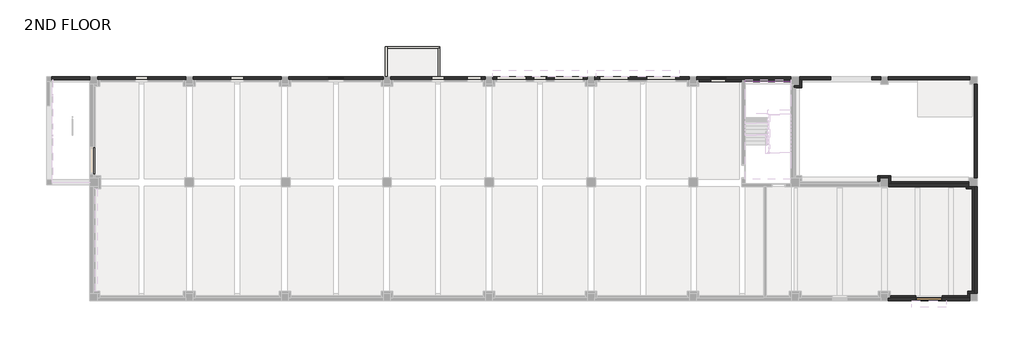
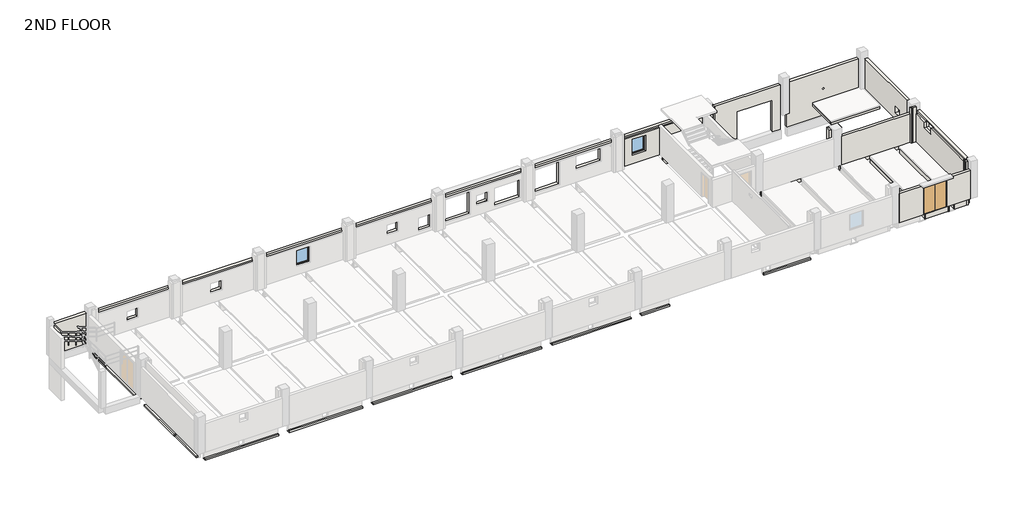
# One storey, part 3 of 7: 46 walls, 2 slabs, 2 windows, 1 door.
"""IFC4 building model written with IfcOpenShell, lengths in millimetres."""

import ifcopenshell
import ifcopenshell.guid

model = None  # the IFC model being written
_history = None  # IfcOwnerHistory: only IFC2X3 demands one
_inside = {}  # id of a spatial element -> (the spatial element, [elements in it])
_under = {}  # id of a project, library or spatial element -> (it, [spatial elements below it])
_declared = {}  # id of a project -> (the project, [libraries it declares])
_typed = {}  # id of a type object -> (the type object, [elements of that type])
_made_of = {}  # id of a material, layer set ... -> (it, [elements and type objects made of it])


def new_model(schema):
    """Start an empty IFC model of exactly this schema.

    Asked for "IFC4X3", IfcOpenShell would pick the latest addendum, in which some entities
    have other attributes; the version numbers below select the first issue.
    IFC2X3 requires an IfcOwnerHistory on every rooted entity: one is made here for all.
    """
    global model, _history
    if schema == "IFC4X3":
        model = ifcopenshell.file(schema_version=(4, 3, 0, 0))
    else:
        model = ifcopenshell.file(schema=schema)
    _inside.clear()
    _under.clear()
    _declared.clear()
    _typed.clear()
    _made_of.clear()
    _history = None
    if model.schema == "IFC2X3":
        org = make("IfcOrganization", Name="unknown")
        user = make(
            "IfcPersonAndOrganization",
            ThePerson=make("IfcPerson", FamilyName="unknown"),
            TheOrganization=org,
        )
        app = make(
            "IfcApplication",
            ApplicationDeveloper=org,
            Version="unknown",
            ApplicationFullName="unknown",
            ApplicationIdentifier="unknown",
        )
        _history = make(
            "IfcOwnerHistory",
            OwningUser=user,
            OwningApplication=app,
            ChangeAction="ADDED",
            CreationDate=0,
        )
    return model


def make(cls, **values):
    """One entity of the class cls with the attributes given. An attribute that is None is left unset."""
    return model.create_entity(
        cls, **{name: value for name, value in values.items() if value is not None}
    )


def rooted(cls, **values):
    """An entity with a GlobalId (a new one), such as an element, a storey or a relation."""
    return make(cls, GlobalId=ifcopenshell.guid.new(), OwnerHistory=_history, **values)


def si_unit(unit_type, name, prefix=None):
    """IfcSIUnit, for example si_unit("LENGTHUNIT", "METRE", prefix="MILLI")."""
    return make("IfcSIUnit", UnitType=unit_type, Prefix=prefix, Name=name)


def assignment(units):
    """IfcUnitAssignment: the units of a project."""
    return None if units is None else make("IfcUnitAssignment", Units=units)


def point(xyz):
    """IfcCartesianPoint."""
    return None if xyz is None else make("IfcCartesianPoint", Coordinates=xyz)


def direction(xyz):
    """IfcDirection."""
    return None if xyz is None else make("IfcDirection", DirectionRatios=xyz)


def frame(location, z_axis=None, x_axis=None):
    """IfcAxis2Placement3D, a coordinate frame: its origin and axes. An axis left out is left unset."""
    return make(
        "IfcAxis2Placement3D",
        Location=point(location),
        Axis=direction(z_axis),
        RefDirection=direction(x_axis),
    )


def frame_2d(location, x_axis=None):
    """IfcAxis2Placement2D, a coordinate frame in the plane: its origin and x axis."""
    return make(
        "IfcAxis2Placement2D", Location=point(location), RefDirection=direction(x_axis)
    )


def origin():
    """The frame at (0, 0, 0) with its axes left unset."""
    return frame((0.0, 0.0, 0.0))


def place(relative_to, where):
    """IfcLocalPlacement: puts the frame where relative to a parent placement (None: the world)."""
    return make(
        "IfcLocalPlacement", PlacementRelTo=relative_to, RelativePlacement=where
    )


def context(
    kind, dimensions, precision=None, world=None, true_north=None, identifier=None
):
    """IfcGeometricRepresentationContext, for example the 3D "Model" context."""
    return make(
        "IfcGeometricRepresentationContext",
        ContextIdentifier=identifier,
        ContextType=kind,
        CoordinateSpaceDimension=dimensions,
        Precision=precision,
        WorldCoordinateSystem=world,
        TrueNorth=true_north,
    )


def project(units=None, contexts=None):
    """IfcProject with its units and contexts."""
    return rooted(
        "IfcProject",
        Name="project",
        RepresentationContexts=contexts,
        UnitsInContext=assignment(units),
    )


def spatial(cls, under=None, at=None, **own):
    """A site, building, storey or space (cls), placed at a placement, below another one or the project."""
    s = rooted(cls, ObjectPlacement=at, **own)
    if under is not None:
        _under.setdefault(under.id(), (under, []))[1].append(s)
    return s


def polyline(points):
    """IfcPolyline through the points."""
    return make("IfcPolyline", Points=[point(p) for p in points])


def circle_curve(where, radius):
    """IfcCircle in the frame where."""
    return make("IfcCircle", Position=where, Radius=radius)


def trimmed(basis, trim1, trim2, sense, master):
    """IfcTrimmedCurve: the piece of a basis curve between two trims."""
    return make(
        "IfcTrimmedCurve",
        BasisCurve=basis,
        Trim1=trim1,
        Trim2=trim2,
        SenseAgreement=sense,
        MasterRepresentation=master,
    )


def segment(curve, same_sense, transition):
    """IfcCompositeCurveSegment."""
    return make(
        "IfcCompositeCurveSegment",
        Transition=transition,
        SameSense=same_sense,
        ParentCurve=curve,
    )


def composite_curve(segments, self_intersect=None):
    """IfcCompositeCurve: segments joined end to end."""
    return make("IfcCompositeCurve", Segments=segments, SelfIntersect=self_intersect)


def outline(outer, holes=None, kind="AREA"):
    """IfcArbitraryClosedProfileDef: a profile drawn as a closed curve; with holes, ...WithVoids."""
    if holes is None:
        return make("IfcArbitraryClosedProfileDef", ProfileType=kind, OuterCurve=outer)
    return make(
        "IfcArbitraryProfileDefWithVoids",
        ProfileType=kind,
        OuterCurve=outer,
        InnerCurves=holes,
    )


def extrude(swept, where, along, depth):
    """IfcExtrudedAreaSolid: the profile swept, set in the frame where, extruded along a direction by depth."""
    return make(
        "IfcExtrudedAreaSolid",
        SweptArea=swept,
        Position=where,
        ExtrudedDirection=direction(along),
        Depth=depth,
    )


def faces_of(points, faces, orient=None, outer=None):
    """IfcFace entities. A face is a list of loops; a loop is a list of indices into points, from 0.

    orient and outer hold one flag for each loop. By default every Orientation is true, the
    first loop of a face is its IfcFaceOuterBound and the others are IfcFaceBound.
    """
    made = []
    for i, loops in enumerate(faces):
        bounds = []
        for j, loop in enumerate(loops):
            is_outer = j == 0 if outer is None else outer[i][j]
            bounds.append(
                make(
                    "IfcFaceOuterBound" if is_outer else "IfcFaceBound",
                    Bound=make("IfcPolyLoop", Polygon=[points[k] for k in loop]),
                    Orientation=True if orient is None else orient[i][j],
                )
            )
        made.append(make("IfcFace", Bounds=bounds))
    return made


def faceted_brep(points, faces, orient=None, outer=None, voids=None):
    """IfcFacetedBrep: a solid bounded by flat faces; with voids (closed shells), ...WithVoids."""
    shared = [point(p) for p in points]
    hull = make("IfcClosedShell", CfsFaces=faces_of(shared, faces, orient, outer))
    if voids is None:
        return make("IfcFacetedBrep", Outer=hull)
    return make(
        "IfcFacetedBrepWithVoids",
        Outer=hull,
        Voids=[
            make(cls, CfsFaces=faces_of(shared, fs, o, b)) for cls, fs, o, b in voids
        ],
    )


def shape(context_of_items, identifier, shape_type, items):
    """IfcShapeRepresentation: the items that make up one representation, for example the "Body"."""
    return make(
        "IfcShapeRepresentation",
        ContextOfItems=context_of_items,
        RepresentationIdentifier=identifier,
        RepresentationType=shape_type,
        Items=items,
    )


def source(mapping_origin, context_of_items, identifier, shape_type, items):
    """IfcRepresentationMap: a shape defined once, which mapped items show again and again."""
    return make(
        "IfcRepresentationMap",
        MappingOrigin=mapping_origin,
        MappedRepresentation=shape(context_of_items, identifier, shape_type, items),
    )


def transform(
    local_origin,
    x_axis=None,
    y_axis=None,
    z_axis=None,
    scale=None,
    scale2=None,
    scale3=None,
    uniform=True,
):
    """IfcCartesianTransformationOperator3D, or its non-uniform kind. x_axis, y_axis, z_axis: its Axis1, 2, 3."""
    if uniform:
        return make(
            "IfcCartesianTransformationOperator3D",
            Axis1=direction(x_axis),
            Axis2=direction(y_axis),
            LocalOrigin=point(local_origin),
            Scale=scale,
            Axis3=direction(z_axis),
        )
    return make(
        "IfcCartesianTransformationOperator3DnonUniform",
        Axis1=direction(x_axis),
        Axis2=direction(y_axis),
        LocalOrigin=point(local_origin),
        Scale=scale,
        Axis3=direction(z_axis),
        Scale2=scale2,
        Scale3=scale3,
    )


def mapped(mapping_source, mapping_target):
    """IfcMappedItem: shows the shape of a source again, moved by a transform."""
    return make(
        "IfcMappedItem", MappingSource=mapping_source, MappingTarget=mapping_target
    )


def made_of(thing, what):
    """Note that an element or type object is made of a material, layer set ...; save() writes the relation."""
    if what is not None:
        _made_of.setdefault(what.id(), (what, []))[1].append(thing)
    return thing


def element(
    cls,
    number,
    at=None,
    inside=None,
    cuts=None,
    type_object=None,
    material=None,
    context=None,
    identifier="Body",
    shape_type=None,
    held_by="IfcProductDefinitionShape",
    body=None,
    shapes=None,
    **own,
):
    """One element of the class cls, such as IfcWall. Its Tag is "e" and its number.

    at: its placement. inside: the storey or other place that contains it. cuts: it is an
    opening in that element (IfcRelVoidsElement). A single representation is given by context,
    identifier, shape_type and body (its items); several are given by shapes. held_by: the class
    of the entity that holds the representations. save() writes the other relations.
    """
    e = rooted(cls, Tag="e%d" % number, ObjectPlacement=at, **own)
    if body is not None:
        shapes = [shape(context, identifier, shape_type, body)]
    if shapes is not None:
        e.Representation = make(held_by, Representations=shapes)
    if inside is not None:
        _inside.setdefault(inside.id(), (inside, []))[1].append(e)
    if cuts is not None:
        rooted(
            "IfcRelVoidsElement", RelatingBuildingElement=cuts, RelatedOpeningElement=e
        )
    if type_object is not None:
        _typed.setdefault(type_object.id(), (type_object, []))[1].append(e)
    return made_of(e, material)


def aggregate(whole, parts):
    """IfcRelAggregates: a whole, such as a stair, and the parts it consists of."""
    return rooted("IfcRelAggregates", RelatingObject=whole, RelatedObjects=parts)


def save(model, path):
    """Write the relations noted so far, then the file.

    IfcRelAggregates (storeys below a building ...), IfcRelContainedInSpatialStructure (elements
    in a storey), IfcRelDefinesByType, IfcRelAssociatesMaterial and IfcRelDeclares: one each for
    every whole, place, type object, material and project.
    """
    for whole, parts in _under.values():
        aggregate(whole, parts)
    for where, things in _inside.values():
        rooted(
            "IfcRelContainedInSpatialStructure",
            RelatedElements=things,
            RelatingStructure=where,
        )
    for kind, things in _typed.values():
        rooted("IfcRelDefinesByType", RelatedObjects=things, RelatingType=kind)
    for what, things in _made_of.values():
        rooted("IfcRelAssociatesMaterial", RelatedObjects=things, RelatingMaterial=what)
    for by, libraries in _declared.values():
        rooted("IfcRelDeclares", RelatingContext=by, RelatedDefinitions=libraries)
    model.write(path)


def plane_surface(at):
    """IfcPlane: the flat surface through the origin of the frame at, square to its z axis."""
    return make("IfcPlane", Position=at)


def revolved_surface(curve, axis_point, axis_direction):
    """IfcSurfaceOfRevolution: the curve turned about the line through axis_point along axis_direction."""
    return make(
        "IfcSurfaceOfRevolution",
        SweptCurve=make("IfcArbitraryOpenProfileDef", ProfileType="CURVE", Curve=curve),
        AxisPosition=make("IfcAxis1Placement", Location=point(axis_point), Axis=direction(axis_direction)),
    )


def advanced_brep(points, edges, surfaces, faces):
    """IfcAdvancedBrep: a solid bounded by faces that lie on surfaces and meet in shared edges.

    An edge is (start, end): straight between two places in points (the first is 0);
    or (start, end, curve); or (start, end, curve, False) where it runs against its curve.
    A face is (place in surfaces, loops), or (place, loops, False) where it looks against
    its surface's normal. A loop lists edges by number (the first is 1), with a minus sign
    where the edge is run from its end to its start. The first loop is the outer one.
    """
    corners = [point(p) for p in points]
    vertices = [make("IfcVertexPoint", VertexGeometry=c) for c in corners]
    made = []
    for start, end, *more in edges:
        made.append(
            make(
                "IfcEdgeCurve",
                EdgeStart=vertices[start],
                EdgeEnd=vertices[end],
                EdgeGeometry=more[0] if more else make("IfcPolyline", Points=[corners[start], corners[end]]),
                SameSense=more[1] if len(more) > 1 else True,
            )
        )
    hull = []
    for where, loops, *sense in faces:
        bounds = []
        for j, loop in enumerate(loops):
            ring = [make("IfcOrientedEdge", EdgeElement=made[abs(k) - 1], Orientation=k > 0) for k in loop]
            bounds.append(
                make(
                    "IfcFaceOuterBound" if j == 0 else "IfcFaceBound",
                    Bound=make("IfcEdgeLoop", EdgeList=ring),
                    Orientation=True,
                )
            )
        hull.append(make("IfcAdvancedFace", Bounds=bounds, FaceSurface=surfaces[where], SameSense=sense[0] if sense else True))
    return make("IfcAdvancedBrep", Outer=make("IfcClosedShell", CfsFaces=hull))


def double_door_steel_c24d22a6(model_context):
    return source(origin(), model_context, "Body", "SolidModel", [
        faceted_brep([(-1035.0, -125.0, 2565.0), (-1035.0, 125.0, 2565.0), (-1035.0, 125.0, 0.0), (-1035.0, -125.0, 0.0), (1035.0, 125.0, 0.0), (1035.0, 125.0, 2565.0), (1005.0, 125.0, 2535.0), (-1005.0, 125.0, 2535.0), (-1005.0, 125.0, 30.0), (1005.0, 125.0, 30.0), (1035.0, -125.0, 0.0), (1035.0, -125.0, 2565.0), (1005.0, -125.0, 30.0), (-1005.0, -125.0, 30.0), (-1005.0, -125.0, 2535.0), (1005.0, -125.0, 2535.0), (-1005.0, -85.0, 2535.0), (-1005.0, -85.0, 30.0), (1005.0, -85.0, 30.0), (1005.0, -85.0, 2535.0), (985.0, -85.0, 2515.0), (985.0, -85.0, 50.0), (-985.0, -85.0, 50.0), (-985.0, -85.0, 2515.0), (-985.0, 85.0, 2515.0), (-985.0, 85.0, 50.0), (985.0, 85.0, 50.0), (1005.0, 85.0, 30.0), (-1005.0, 85.0, 30.0), (-1005.0, 85.0, 2535.0), (1005.0, 85.0, 2535.0), (985.0, 85.0, 2515.0)], [[[0, 1, 2, 3]], [[4, 2, 1, 5], [6, 7, 8, 9]], [[3, 2, 4, 10]], [[11, 0, 3, 10], [12, 13, 14, 15]], [[16, 14, 13, 17]], [[17, 13, 12, 18]], [[16, 17, 18, 19], [20, 21, 22, 23]], [[24, 23, 22, 25]], [[25, 22, 21, 26]], [[27, 28, 29, 30], [31, 24, 25, 26]], [[7, 29, 28, 8]], [[8, 28, 27, 9]], [[10, 4, 5, 11]], [[9, 27, 30, 6]], [[18, 12, 15, 19]], [[26, 21, 20, 31]], [[11, 5, 1, 0]], [[19, 15, 14, 16]], [[31, 20, 23, 24]], [[6, 30, 29, 7]]]),
        extrude(outline(polyline([(1005.0, 85.0), (0.0, 85.0), (0.0, 125.0), (1005.0, 125.0), (1005.0, 85.0)])), frame((0.0, 0.0, 30.0), z_axis=(0.0, 0.0, 1.0), x_axis=(1.0, 0.0, 0.0)), (0.0, 0.0, 1.0), 2505.0),
        extrude(outline(polyline([(0.0, 85.0), (-1005.0, 85.0), (-1005.0, 125.0), (0.0, 125.0), (0.0, 85.0)])), frame((0.0, 0.0, 30.0), z_axis=(0.0, 0.0, 1.0), x_axis=(1.0, 0.0, 0.0)), (0.0, 0.0, 1.0), 2505.0),
    ])


def fixed_window_c6e05aa5(model_context):
    return source(origin(), model_context, "Body", "SweptSolid", [
        extrude(outline(polyline([(-550.0, 3.0), (550.0, 3.0), (550.0, -3.0), (-550.0, -3.0), (-550.0, 3.0)])), frame((0.0, 0.0, 850.0), z_axis=(0.0, 0.0, 1.0), x_axis=(1.0, 0.0, 0.0)), (0.0, 0.0, 1.0), 1400.0),
        extrude(outline(polyline([(2300.0, -600.0), (800.0, -600.0), (800.0, 600.0), (2300.0, 600.0), (2300.0, -600.0)]), holes=[polyline([(2250.0, -550.0), (2250.0, 550.0), (850.0, 550.0), (850.0, -550.0), (2250.0, -550.0)])]), frame((0.0, -75.0, 0.0), z_axis=(0.0, 1.0, 0.0), x_axis=(0.0, 0.0, 1.0)), (0.0, 0.0, 1.0), 150.0),
    ])


model = new_model("IFC4")

# Units and contexts
model_context = context("Model", 3, world=origin())
ifc_project = project(units=[si_unit("LENGTHUNIT", "METRE", prefix="MILLI")], contexts=[model_context])

# Site, building, storey
site = spatial("IfcSite", under=ifc_project)
building = spatial("IfcBuilding", under=site)
storey = spatial("IfcBuildingStorey", under=building, Name="2ND FLOOR", Elevation=10600.0)

# Door
placement = place(None, origin())
double_door_steel_shape = double_door_steel_c24d22a6(model_context)
element("IfcDoor", 1, ObjectType="Double Door_Steel : H_DR_AR B12_Door_Double_W2100xH2580_No FR_SD-5", at=placement, inside=storey, context=model_context, shape_type="MappedRepresentation", body=[
    mapped(double_door_steel_shape, transform((65500.0, -17175.0, 10600.0), x_axis=(-1.0, 0.0, 0.0), y_axis=(0.0, -1.0, 0.0), z_axis=(0.0, 0.0, 1.0))),
])

# Slabs
element("IfcSlab", 2, ObjectType="H_WA_AR_B02_Int Wall_2L Gypsum_Insulationl_T154(Mirror)", at=placement, inside=storey, context=model_context, shape_type="Brep", body=[
    faceted_brep([(264.0, -8514.0, 9736.0), (264.0, -13136.0, 9736.0), (114.0, -13136.0, 9736.0), (-40.0, -13136.0, 9736.0), (-40.0, -8514.0, 9736.0), (114.0, -8514.0, 9736.0), (110.0, -8514.0, 9890.0), (-40.0, -8514.0, 9890.0), (-40.0, -13136.0, 9890.0), (110.0, -13136.0, 9890.0), (264.0, -8514.0, 9755.0), (264.0, -13136.0, 9755.0), (110.0, -8514.0, 9755.0), (110.0, -13136.0, 9755.0), (114.0, -13136.0, 9755.0), (-40.0, -13136.0, 9755.0)], [[[0, 1, 2, 3, 4, 5]], [[6, 7, 8, 9]], [[1, 0, 10, 11]], [[0, 5, 4, 7, 6, 12, 10]], [[13, 12, 6, 9]], [[12, 13, 14, 11, 10]], [[3, 2, 1, 11, 14, 13, 9, 8, 15]], [[4, 3, 15, 8, 7]]]),
    faceted_brep([(264.0, -16536.0, 9736.0), (114.0, -16536.0, 9736.0), (-40.0, -16536.0, 9736.0), (-40.0, -13264.0, 9736.0), (114.0, -13264.0, 9736.0), (264.0, -13264.0, 9736.0), (-40.0, -13264.0, 9890.0), (-40.0, -16536.0, 9890.0), (110.0, -16536.0, 9890.0), (110.0, -13264.0, 9890.0), (264.0, -16536.0, 9755.0), (110.0, -16536.0, 9755.0), (-40.0, -13264.0, 9755.0), (110.0, -13264.0, 9755.0), (264.0, -13264.0, 9755.0), (114.0, -13264.0, 9755.0)], [[[0, 1, 2, 3, 4, 5]], [[6, 7, 8, 9]], [[2, 1, 0, 10, 11, 8, 7]], [[3, 2, 7, 6, 12]], [[9, 8, 11, 13]], [[14, 15, 13, 11, 10]], [[5, 4, 3, 12, 6, 9, 13, 15, 14]], [[0, 5, 14, 10]]]),
    faceted_brep([(264.0, -7486.0, 9736.0), (114.0, -7486.0, 9736.0), (-40.0, -7486.0, 9736.0), (-40.0, -464.0, 9736.0), (114.0, -464.0, 9736.0), (264.0, -464.0, 9736.0), (-40.0, -464.0, 9890.0), (-40.0, -7486.0, 9890.0), (110.0, -7486.0, 9890.0), (110.0, -464.0, 9890.0), (264.0, -7486.0, 9755.0), (110.0, -7486.0, 9755.0), (110.0, -464.0, 9755.0), (264.0, -464.0, 9755.0)], [[[0, 1, 2, 3, 4, 5]], [[6, 7, 8, 9]], [[2, 1, 0, 10, 11, 8, 7]], [[3, 2, 7, 6]], [[5, 4, 3, 6, 9, 12, 13]], [[0, 5, 13, 10]], [[11, 12, 9, 8]], [[12, 11, 10, 13]]]),
])
element("IfcSlab", 3, ObjectType="H_WA_AR_B02_Int Wall_2L Gypsum_Insulationl_T154(Mirror)", at=placement, inside=storey, context=model_context, shape_type="Brep", body=[
    faceted_brep([(464.0, -17040.0, 9636.0), (464.0, -16886.0, 9636.0), (464.0, -16736.0, 9636.0), (7036.0, -16736.0, 9636.0), (7036.0, -16886.0, 9636.0), (7036.0, -17040.0, 9636.0), (464.0, -17040.0, 9790.0), (7036.0, -17040.0, 9790.0), (7036.0, -16890.0, 9790.0), (464.0, -16890.0, 9790.0), (464.0, -16890.0, 9655.0), (464.0, -16736.0, 9655.0), (7036.0, -16736.0, 9655.0), (7036.0, -16890.0, 9655.0)], [[[0, 1, 2, 3, 4, 5]], [[6, 7, 8, 9]], [[2, 1, 0, 6, 9, 10, 11]], [[3, 2, 11, 12]], [[5, 4, 3, 12, 13, 8, 7]], [[0, 5, 7, 6]], [[13, 10, 9, 8]], [[10, 13, 12, 11]]]),
    faceted_brep([(14536.0, -16736.0, 9636.0), (14536.0, -16886.0, 9636.0), (14536.0, -17040.0, 9636.0), (7964.0, -17040.0, 9636.0), (7964.0, -16886.0, 9636.0), (7964.0, -16736.0, 9636.0), (7964.0, -17040.0, 9790.0), (14536.0, -17040.0, 9790.0), (14536.0, -16890.0, 9790.0), (7964.0, -16890.0, 9790.0), (14536.0, -16736.0, 9655.0), (14536.0, -16890.0, 9655.0), (7964.0, -16890.0, 9655.0), (7964.0, -16736.0, 9655.0)], [[[0, 1, 2, 3, 4, 5]], [[6, 7, 8, 9]], [[2, 1, 0, 10, 11, 8, 7]], [[3, 2, 7, 6]], [[5, 4, 3, 6, 9, 12, 13]], [[0, 5, 13, 10]], [[11, 12, 9, 8]], [[12, 11, 10, 13]]]),
    faceted_brep([(23464.0, -16736.0, 9636.0), (30536.0, -16736.0, 9636.0), (30536.0, -16886.0, 9636.0), (23464.0, -16886.0, 9636.0), (23464.0, -16736.0, 9655.0), (23464.0, -16886.0, 9655.0), (30536.0, -16736.0, 9655.0), (30536.0, -16886.0, 9655.0)], [[[0, 1, 2, 3]], [[4, 0, 3, 5]], [[1, 0, 4, 6]], [[2, 1, 6, 7]], [[6, 4, 5, 7]], [[3, 2, 7, 5]]]),
    faceted_brep([(31464.0, -16736.0, 9636.0), (38536.0, -16736.0, 9636.0), (38536.0, -16886.0, 9636.0), (31464.0, -16886.0, 9636.0), (31464.0, -16736.0, 9655.0), (31464.0, -16886.0, 9655.0), (38536.0, -16736.0, 9655.0), (38536.0, -16886.0, 9655.0)], [[[0, 1, 2, 3]], [[4, 0, 3, 5]], [[1, 0, 4, 6]], [[1, 6, 7, 2]], [[6, 4, 5, 7]], [[3, 2, 7, 5]]]),
    faceted_brep([(22536.0, -17040.0, 9636.0), (15464.0, -17040.0, 9636.0), (15464.0, -16886.0, 9636.0), (15464.0, -16736.0, 9636.0), (22536.0, -16736.0, 9636.0), (22536.0, -16886.0, 9636.0), (15464.0, -17040.0, 9790.0), (22536.0, -17040.0, 9790.0), (22536.0, -16890.0, 9790.0), (15464.0, -16890.0, 9790.0), (15464.0, -16890.0, 9655.0), (15464.0, -16736.0, 9655.0), (22536.0, -16736.0, 9655.0), (22536.0, -16890.0, 9655.0)], [[[0, 1, 2, 3, 4, 5]], [[6, 7, 8, 9]], [[1, 0, 7, 6]], [[3, 2, 1, 6, 9, 10, 11]], [[4, 3, 11, 12]], [[0, 5, 4, 12, 13, 8, 7]], [[13, 10, 9, 8]], [[10, 13, 12, 11]]]),
    faceted_brep([(41975.0, -16736.0, 9636.0), (41975.0, -16886.0, 9636.0), (41975.0, -17040.0, 9636.0), (39464.0, -17040.0, 9636.0), (39464.0, -16886.0, 9636.0), (39464.0, -16736.0, 9636.0), (39464.0, -17040.0, 9790.0), (41975.0, -17040.0, 9790.0), (41975.0, -16890.0, 9790.0), (39464.0, -16890.0, 9790.0), (41975.0, -16736.0, 9655.0), (41975.0, -16890.0, 9655.0), (39464.0, -16890.0, 9655.0), (39464.0, -16736.0, 9655.0)], [[[0, 1, 2, 3, 4, 5]], [[6, 7, 8, 9]], [[2, 1, 0, 10, 11, 8, 7]], [[3, 2, 7, 6]], [[5, 4, 3, 6, 9, 12, 13]], [[0, 5, 13, 10]], [[11, 12, 9, 8]], [[12, 11, 10, 13]]]),
    faceted_brep([(50343.0, -16736.0, 9636.0), (54536.0, -16736.0, 9636.0), (54536.0, -16886.0, 9636.0), (54536.0, -17040.0, 9636.0), (50343.0, -17040.0, 9636.0), (50343.0, -16886.0, 9636.0), (50343.0, -17040.0, 9790.0), (54536.0, -17040.0, 9790.0), (54536.0, -16890.0, 9790.0), (50343.0, -16890.0, 9790.0), (50343.0, -16736.0, 9655.0), (54536.0, -16736.0, 9655.0), (54536.0, -16890.0, 9655.0), (50343.0, -16890.0, 9655.0)], [[[0, 1, 2, 3, 4, 5]], [[6, 7, 8, 9]], [[1, 0, 10, 11]], [[3, 2, 1, 11, 12, 8, 7]], [[4, 3, 7, 6]], [[0, 5, 4, 6, 9, 13, 10]], [[12, 13, 9, 8]], [[13, 12, 11, 10]]]),
    faceted_brep([(23464.0, -17040.0, 9790.0), (30536.0, -17040.0, 9790.0), (30536.0, -16890.0, 9790.0), (23464.0, -16890.0, 9790.0), (23464.0, -16890.0, 9655.0), (23464.0, -17040.0, 9655.0), (30536.0, -17040.0, 9655.0), (30536.0, -16890.0, 9655.0)], [[[0, 1, 2, 3]], [[0, 3, 4, 5]], [[1, 6, 7, 2]], [[1, 0, 5, 6]], [[3, 2, 7, 4]], [[5, 4, 7, 6]]]),
    faceted_brep([(31464.0, -17040.0, 9790.0), (38536.0, -17040.0, 9790.0), (38536.0, -16890.0, 9790.0), (31464.0, -16890.0, 9790.0), (31464.0, -17040.0, 9655.0), (38536.0, -17040.0, 9655.0), (31464.0, -16890.0, 9655.0), (38536.0, -16890.0, 9655.0)], [[[0, 1, 2, 3]], [[1, 0, 4, 5]], [[0, 3, 6, 4]], [[2, 1, 5, 7]], [[3, 2, 7, 6]], [[5, 4, 6, 7]]]),
])

# Walls
element("IfcWall", 4, ObjectType="H_WA_AR B02_Ext Wall RC-AG_T250_W1", at=placement, inside=storey, context=model_context, shape_type="SweptSolid", body=[
    extrude(outline(polyline([(10600.0, 300.0), (10600.0, 7200.0), (13300.0, 7200.0), (13300.0, 300.0), (10600.0, 300.0)]), holes=[polyline([(12450.0, 3250.0), (12450.0, 4250.0), (11550.0, 4250.0), (11550.0, 3250.0), (12450.0, 3250.0)])]), frame((0.0, 50.0, 0.0), z_axis=(0.0, 1.0, 0.0), x_axis=(0.0, 0.0, 1.0)), (0.0, 0.0, 1.0), 250.0),
])
element("IfcWall", 5, ObjectType="H_WA_AR B02_Ext Wall RC-AG_T250_W1", at=placement, inside=storey, context=model_context, shape_type="SweptSolid", body=[
    extrude(outline(polyline([(10600.0, 7800.0), (10600.0, 14700.0), (13300.0, 14700.0), (13300.0, 7800.0), (10600.0, 7800.0)]), holes=[polyline([(12450.0, 10750.0), (12450.0, 11750.0), (11550.0, 11750.0), (11550.0, 10750.0), (12450.0, 10750.0)])]), frame((0.0, 50.0, 0.0), z_axis=(0.0, 1.0, 0.0), x_axis=(0.0, 0.0, 1.0)), (0.0, 0.0, 1.0), 250.0),
])
element("IfcWall", 6, ObjectType="H_WA_AR B02_Ext Wall RC-AG_T250_W1", at=placement, inside=storey, context=model_context, shape_type="SweptSolid", body=[
    extrude(outline(polyline([(10600.0, 15299.9999999), (10600.0, 22700.0), (13300.0, 22700.0), (13300.0, 15299.9999999), (10600.0, 15299.9999999)]), holes=[polyline([(11400.0, 19599.9999999), (11400.0, 18399.9999999), (12900.0, 18399.9999999), (12900.0, 19599.9999999), (11400.0, 19599.9999999)])]), frame((0.0, 50.0, 0.0), z_axis=(0.0, 1.0, 0.0), x_axis=(0.0, 0.0, 1.0)), (0.0, 0.0, 1.0), 250.0),
])
element("IfcWall", 7, ObjectType="H_WA_AR B02_Ext Wall RC-AG_T250_W1", at=placement, inside=storey, context=model_context, shape_type="SweptSolid", body=[
    extrude(outline(polyline([(10600.0, 23300.0), (10600.0, 30700.0), (13300.0, 30700.0), (13300.0, 23300.0), (10600.0, 23300.0)]), holes=[polyline([(12150.0, 29300.0), (12150.0, 30400.0), (10900.0, 30400.0), (10900.0, 29300.0), (12150.0, 29300.0)]), polyline([(12450.0, 26500.0), (12450.0, 27500.0), (11550.0, 27500.0), (11550.0, 26500.0), (12450.0, 26500.0)])]), frame((0.0, 50.0, 0.0), z_axis=(0.0, 1.0, 0.0), x_axis=(0.0, 0.0, 1.0)), (0.0, 0.0, 1.0), 250.0),
])
element("IfcWall", 8, ObjectType="H_WA_AR B02_Ext Wall RC-AG_T250_W1", at=placement, inside=storey, context=model_context, shape_type="SweptSolid", body=[
    extrude(outline(polyline([(10600.0, 31300.0), (10600.0, 38700.0), (13300.0, 38700.0), (13300.0, 31300.0), (10600.0, 31300.0)]), holes=[polyline([(12600.0, 36100.0), (12600.0, 38400.0), (10900.0, 38400.0), (10900.0, 36100.0), (12600.0, 36100.0)]), polyline([(13050.0, 31600.0), (13050.0, 33900.0), (10900.0, 33900.0), (10900.0, 31600.0), (13050.0, 31600.0)]), polyline([(12450.0, 34500.0), (12450.0, 35500.0), (11550.0, 35500.0), (11550.0, 34500.0), (12450.0, 34500.0)])]), frame((0.0, 50.0, 0.0), z_axis=(0.0, 1.0, 0.0), x_axis=(0.0, 0.0, 1.0)), (0.0, 0.0, 1.0), 250.0),
])
element("IfcWall", 9, ObjectType="H_WA_AR B02_Ext Wall RC-AG_T250_W1", at=placement, inside=storey, context=model_context, shape_type="SweptSolid", body=[
    extrude(outline(polyline([(10600.0, 39300.0), (10600.0, 46700.0), (13300.0, 46700.0), (13300.0, 39300.0), (10600.0, 39300.0)]), holes=[composite_curve([segment(trimmed(circle_curve(frame_2d((12955.0, 46436.0)), 25.0), [point((12955.0, 46411.0))], [point((12955.0, 46461.0))], True, "CARTESIAN"), True, "CONTINUOUS"), segment(trimmed(circle_curve(frame_2d((12955.0, 46436.0)), 25.0), [point((12955.0, 46461.0))], [point((12955.0, 46411.0))], True, "CARTESIAN"), True, "CONTINUOUS")], self_intersect=False), polyline([(13050.0, 43400.0), (13050.0, 45600.0), (11800.0, 45600.0), (11800.0, 43400.0), (13050.0, 43400.0)]), polyline([(10900.0, 39700.0195059), (13050.0, 39700.0195059), (13050.0, 41900.0195059), (10900.0, 41900.0195059), (10900.0, 39700.0195059)])]), frame((0.0, 50.0, 0.0), z_axis=(0.0, 1.0, 0.0), x_axis=(0.0, 0.0, 1.0)), (0.0, 0.0, 1.0), 250.0),
])
element("IfcWall", 10, ObjectType="H_WA_AR B02_Ext Wall RC-AG_T250_W1", at=placement, inside=storey, context=model_context, shape_type="Brep", body=[
    faceted_brep([(47300.0, 50.0, 10600.0), (50825.0, 50.0, 10600.0), (51075.0, 50.0, 10600.0), (54650.0, 50.0, 10600.0), (54650.0, 50.0, 13300.0), (51075.0, 50.0, 13300.0), (50825.0, 50.0, 13300.0), (47300.0, 50.0, 13300.0), (49575.0, 50.0, 11400.0), (48375.0, 50.0, 11400.0), (48375.0, 50.0, 12900.0), (49575.0, 50.0, 12900.0), (47300.0, 300.0, 10600.0), (47300.0, 300.0, 13300.0), (54650.0, 300.0, 13300.0), (54650.0, 300.0, 10600.0), (49575.0, 300.0, 11400.0), (49575.0, 300.0, 12900.0), (48375.0, 300.0, 12900.0), (48375.0, 300.0, 11400.0)], [[[0, 1, 2, 3, 4, 5, 6, 7], [8, 9, 10, 11]], [[12, 13, 14, 15], [16, 17, 18, 19]], [[3, 2, 1, 0, 12, 15]], [[4, 3, 15, 14]], [[7, 6, 5, 4, 14, 13]], [[0, 7, 13, 12]], [[17, 16, 8, 11]], [[18, 17, 11, 10]], [[19, 18, 10, 9]], [[16, 19, 9, 8]]]),
])
element("IfcWall", 11, ObjectType="H_WA_AR B02_Ext Wall RC-AG_T250_W1", at=placement, inside=storey, context=model_context, shape_type="Brep", body=[
    faceted_brep([(61000.0, 50.0, 12100.0), (61000.0, 50.0, 9100.0), (61700.0, 50.0, 9100.0), (61700.0, 50.0, 13300.0), (55350.0, 50.0, 13300.0), (55350.0, 50.0, 9100.0), (57800.0, 50.0, 9100.0), (57800.0, 50.0, 12100.0), (61700.0, 300.0, 9100.0), (61000.0, 300.0, 9100.0), (61000.0, 300.0, 12100.0), (57800.0, 300.0, 12100.0), (57800.0, 300.0, 9100.0), (55350.0, 300.0, 9100.0), (55350.0, 300.0, 10600.0), (55350.0, 300.0, 13300.0), (61700.0, 300.0, 13300.0), (61700.0, 300.0, 10600.0)], [[[0, 1, 2, 3, 4, 5, 6, 7]], [[8, 9, 10, 11, 12, 13, 14, 15, 16, 17]], [[6, 5, 13, 12]], [[2, 1, 9, 8]], [[3, 2, 8, 17, 16]], [[4, 3, 16, 15]], [[5, 4, 15, 14, 13]], [[12, 11, 7, 6]], [[10, 9, 1, 0]], [[11, 10, 0, 7]]]),
])
element("IfcWall", 12, ObjectType="H_WA_AR B02_Ext Wall RC-AG_T250_W1", at=placement, inside=storey, context=model_context, shape_type="AdvancedBrep", body=[
    advanced_brep(
    [(62300.0, 50.0, 9100.0), (68700.0, 50.0, 9100.0), (68700.0, 50.0, 13300.0), (62300.0, 50.0, 13300.0), (65618.0, 50.0, 11600.0), (65468.0, 50.0, 11600.0), (68700.0, 300.0, 9100.0), (62300.0, 300.0, 9100.0), (62300.0, 300.0, 10600.0), (62300.0, 300.0, 13300.0), (68700.0, 300.0, 13300.0), (68700.0, 300.0, 10600.0), (65468.0, 300.0, 11600.0), (65618.0, 300.0, 11600.0)],
    [
        (0, 1),
        (1, 2),
        (2, 3),
        (3, 0),
        (4, 5, circle_curve(frame((65543.0, 50.0, 11600.0), z_axis=(0.0, 1.0, 0.0), x_axis=(1.0, 0.0, 0.0)), 75.0)),
        (5, 4, circle_curve(frame((65543.0, 50.0, 11600.0), z_axis=(0.0, 1.0, 0.0), x_axis=(1.0, 0.0, 0.0)), 75.0)),
        (6, 7),
        (7, 8),
        (8, 9),
        (9, 10),
        (10, 11),
        (11, 6),
        (12, 13, circle_curve(frame((65543.0, 300.0, 11600.0), z_axis=(0.0, -1.0, 0.0), x_axis=(1.0, 0.0, 0.0)), 75.0)),
        (13, 12, circle_curve(frame((65543.0, 300.0, 11600.0), z_axis=(0.0, -1.0, 0.0), x_axis=(1.0, 0.0, 0.0)), 75.0)),
        (0, 7),
        (6, 1),
        (10, 2),
        (9, 3),
        (12, 5),
        (4, 13),
    ],
    [
        plane_surface(frame((62300.0, 50.0, 9100.0), z_axis=(0.0, -1.0, 0.0), x_axis=(1.0, 0.0, 0.0))),
        plane_surface(frame((62300.0, 300.0, 9100.0), z_axis=(0.0, 1.0, 0.0), x_axis=(-1.0, 0.0, 0.0))),
        plane_surface(frame((62300.0, 50.0, 9100.0), z_axis=(0.0, 0.0, -1.0), x_axis=(0.0, 1.0, 0.0))),
        plane_surface(frame((68700.0, 50.0, 9100.0), z_axis=(1.0, 0.0, 0.0), x_axis=(0.0, 1.0, 0.0))),
        plane_surface(frame((68700.0, 50.0, 13300.0), z_axis=(0.0, 0.0, 1.0), x_axis=(0.0, 1.0, 0.0))),
        plane_surface(frame((62300.0, 50.0, 13300.0), z_axis=(-1.0, 0.0, 0.0), x_axis=(0.0, 1.0, 0.0))),
        revolved_surface(polyline([(65618.0, 50.0, 11600.0), (65618.0, 300.0, 11600.0)]), (65543.0, 50.0, 11600.0), (0.0, -1.0, 0.0)),
    ],
    [
        (0, [[1, 2, 3, 4], [5, 6]]),
        (1, [[7, 8, 9, 10, 11, 12], [13, 14]]),
        (2, [[-1, 15, -7, 16]]),
        (3, [[-2, -16, -12, -11, 17]]),
        (4, [[-3, -17, -10, 18]]),
        (5, [[-4, -18, -9, -8, -15]]),
        (6, [[-13, 19, -5, 20]]),
        (6, [[-14, -20, -6, -19]]),
    ],
),
])
element("IfcWall", 13, ObjectType="H_WA_AR B02_Ext Wall RC-AG_T250_W1", at=placement, inside=storey, context=model_context, shape_type="SweptSolid", body=[
    extrude(outline(polyline([(-300.0, 10600.0), (-7650.0, 10600.0), (-7650.0, 13400.0), (-300.0, 13400.0), (-300.0, 10600.0)]), holes=[polyline([(-5050.0, 11800.0), (-5650.0, 11800.0), (-5650.0, 11200.0), (-5050.0, 11200.0), (-5050.0, 11800.0)])]), frame((69050.0, 0.0, 0.0), z_axis=(1.0, 0.0, 0.0), x_axis=(0.0, 1.0, 0.0)), (0.0, 0.0, 1.0), 250.0),
])
element("IfcWall", 14, ObjectType="H_WA_AR B02_Ext Wall RC-AG_T250_W1", at=placement, inside=storey, context=model_context, shape_type="SweptSolid", body=[
    extrude(outline(polyline([(-8350.0, 10600.0), (-16700.0, 10600.0), (-16700.0, 13400.0), (-8350.0, 13400.0), (-8350.0, 10600.0)]), holes=[polyline([(-9800.0, 13300.0), (-10800.0, 13300.0), (-10800.0, 12700.0), (-9800.0, 12700.0), (-9800.0, 13300.0)])]), frame((69050.0, 0.0, 0.0), z_axis=(1.0, 0.0, 0.0), x_axis=(0.0, 1.0, 0.0)), (0.0, 0.0, 1.0), 250.0),
])
element("IfcWall", 15, ObjectType="H_WA_AR B02_Ext Wall RC-AG_T250_W1", at=placement, inside=storey, context=model_context, shape_type="SweptSolid", body=[
    extrude(outline(polyline([(13300.0, 62300.0), (10600.0, 62300.0), (10600.0, 64450.0), (13180.0, 64450.0), (13180.0, 66550.0), (10600.0, 66550.0), (10600.0, 68700.0), (13300.0, 68700.0), (13300.0, 62300.0)])), frame((0.0, -17300.0, 0.0), z_axis=(0.0, 1.0, 0.0), x_axis=(0.0, 0.0, 1.0)), (0.0, 0.0, 1.0), 250.0),
])
element("IfcWall", 16, ObjectType="H_WA_AR B02_Ext Wall RC-AG_T250_W1", at=placement, inside=storey, context=model_context, shape_type="Brep", body=[
    faceted_brep([(-300.0, 300.0, 10550.0), (-3300.0, 300.0, 10550.0), (-3300.0, 300.0, 10600.0), (-3300.0, 300.0, 13450.0), (-300.0, 300.0, 13450.0), (-300.0, 300.0, 10600.0), (-300.0, 50.0, 10550.0), (-300.0, 50.0, 13450.0), (-3300.0, 50.0, 13450.0), (-3300.0, 50.0, 10550.0)], [[[0, 1, 2, 3, 4, 5]], [[6, 7, 8, 9]], [[1, 0, 6, 9]], [[3, 2, 1, 9, 8]], [[4, 3, 8, 7]], [[0, 5, 4, 7, 6]]]),
])
element("IfcWall", 17, ObjectType="H_WA_AR B02_Int Wall RC-AG_T250_W2", at=placement, inside=storey, context=model_context, shape_type="SweptSolid", body=[
    extrude(outline(polyline([(68600.0, -8350.0), (62350.0, -8350.0), (62350.0, -8100.0), (68600.0, -8100.0), (68600.0, -8350.0)])), frame((0.0, 0.0, 10600.0), z_axis=(0.0, 0.0, 1.0), x_axis=(1.0, 0.0, 0.0)), (0.0, 0.0, 1.0), 2700.0),
])
element("IfcWall", 18, ObjectType="H_WA_AR B02_Ext Wall RC-AG_T150", at=placement, inside=storey, context=model_context, shape_type="Brep", body=[
    faceted_brep([(22850.0, 2650.0, 9300.0), (22850.0, 2350.0, 9300.0), (22850.0, 300.0, 9300.0), (22850.0, 300.0, 9900.0), (22850.0, 2650.0, 9900.0), (23000.0, 2650.0, 9300.0), (23000.0, 2650.0, 9900.0), (23000.0, 2500.0, 9900.0), (23000.0, 300.0, 9900.0), (23000.0, 300.0, 9300.0), (23000.0, 2500.0, 9300.0)], [[[0, 1, 2, 3, 4]], [[5, 6, 7, 8, 9, 10]], [[2, 1, 0, 5, 10, 9]], [[3, 2, 9, 8]], [[4, 3, 8, 7, 6]], [[0, 4, 6, 5]]]),
])
element("IfcWall", 19, ObjectType="H_WA_AR B02_Ext Wall RC-AG_T150", at=placement, inside=storey, context=model_context, shape_type="Brep", body=[
    faceted_brep([(27150.0, 2650.0, 9300.0), (26850.0, 2650.0, 9300.0), (23150.0, 2650.0, 9300.0), (23000.0, 2650.0, 9300.0), (23000.0, 2650.0, 9900.0), (27150.0, 2650.0, 9900.0), (27150.0, 2500.0, 9300.0), (27150.0, 2500.0, 9900.0), (27000.0, 2500.0, 9900.0), (23000.0, 2500.0, 9900.0), (23000.0, 2500.0, 9300.0), (27000.0, 2500.0, 9300.0)], [[[0, 1, 2, 3, 4, 5]], [[6, 7, 8, 9, 10, 11]], [[3, 2, 1, 0, 6, 11, 10]], [[5, 4, 9, 8, 7]], [[4, 3, 10, 9]], [[0, 5, 7, 6]]]),
])
element("IfcWall", 20, ObjectType="H_WA_AR B02_Ext Wall RC-AG_T150", at=placement, inside=storey, context=model_context, shape_type="Brep", body=[
    faceted_brep([(27150.0, 300.0, 9300.0), (27150.0, 2350.0, 9300.0), (27150.0, 2500.0, 9300.0), (27150.0, 2500.0, 9900.0), (27150.0, 300.0, 9900.0), (27000.0, 300.0, 9300.0), (27000.0, 300.0, 9900.0), (27000.0, 2500.0, 9900.0), (27000.0, 2500.0, 9300.0)], [[[0, 1, 2, 3, 4]], [[5, 6, 7, 8]], [[2, 1, 0, 5, 8]], [[4, 3, 7, 6]], [[0, 4, 6, 5]], [[3, 2, 8, 7]]]),
])
element("IfcWall", 21, ObjectType="H_WA_AR_B02_Ext Wall_Concrete Lintel_T190", at=placement, inside=storey, context=model_context, shape_type="Brep", body=[
    faceted_brep([(68900.0, -2660.0, 10260.0), (64790.0, -2660.0, 10260.0), (64600.0, -2660.0, 10260.0), (64600.0, -2660.0, 10450.0), (64790.0, -2660.0, 10450.0), (68900.0, -2660.0, 10450.0), (68900.0, -2850.0, 10260.0), (68900.0, -2850.0, 10450.0), (64600.0, -2850.0, 10450.0), (64600.0, -2850.0, 10260.0)], [[[0, 1, 2, 3, 4, 5]], [[6, 7, 8, 9]], [[2, 1, 0, 6, 9]], [[5, 4, 3, 8, 7]], [[0, 5, 7, 6]], [[3, 2, 9, 8]]]),
])
element("IfcWall", 22, ObjectType="H_WA_AR_B02_Ext Wall_Concrete Lintel_T190", at=placement, inside=storey, context=model_context, shape_type="SweptSolid", body=[
    extrude(outline(polyline([(64790.0, 50.0), (64790.0, -2660.0), (64600.0, -2660.0), (64600.0, 50.0), (64790.0, 50.0)])), frame((0.0, 0.0, 10260.0), z_axis=(0.0, 0.0, 1.0), x_axis=(1.0, 0.0, 0.0)), (0.0, 0.0, 1.0), 190.0),
])
element("IfcWall", 23, ObjectType="H_WA_AR B02_Ext Wall DY-IN_T154", at=placement, inside=storey, context=model_context, shape_type="SweptSolid", body=[
    extrude(outline(polyline([(62464.0, -17040.0), (62464.0, -16886.0), (64450.0, -16886.0), (64450.0, -17040.0), (62464.0, -17040.0)])), frame((0.0, 0.0, 10600.0), z_axis=(0.0, 0.0, 1.0), x_axis=(1.0, 0.0, 0.0)), (0.0, 0.0, 1.0), 2536.0),
    extrude(outline(polyline([(68536.0, -16886.0), (68536.0, -17040.0), (66550.0, -17040.0), (66550.0, -16886.0), (68536.0, -16886.0)])), frame((0.0, 0.0, 10600.0), z_axis=(0.0, 0.0, 1.0), x_axis=(1.0, 0.0, 0.0)), (0.0, 0.0, 1.0), 2536.0),
])
element("IfcWall", 24, ObjectType="H_WA_AR B02_Ext Wall DY-IN_T154", at=placement, inside=storey, context=model_context, shape_type="Brep", body=[
    faceted_brep([(68886.0, -8360.0, 10600.0), (68886.0, -8514.0, 10600.0), (68886.0, -16536.0, 10600.0), (68886.0, -16536.0, 13236.0), (68886.0, -10800.0, 13236.0), (68886.0, -10800.0, 12700.0), (68886.0, -9800.0, 12700.0), (68886.0, -9800.0, 13236.0), (68886.0, -8514.0, 13236.0), (68886.0, -8514.0, 13255.0), (68886.0, -8360.0, 13255.0), (69040.0, -16536.0, 10600.0), (69040.0, -8360.0, 10600.0), (69040.0, -8360.0, 13255.0), (69040.0, -8514.0, 13255.0), (69040.0, -8514.0, 13236.0), (69040.0, -9800.0, 13236.0), (69040.0, -9800.0, 12700.0), (69040.0, -10800.0, 12700.0), (69040.0, -10800.0, 13236.0), (69040.0, -16536.0, 13236.0), (68890.0, -8360.0, 13255.0), (68890.0, -8514.0, 13255.0)], [[[0, 1, 2, 3, 4, 5, 6, 7, 8, 9, 10]], [[11, 12, 13, 14, 15, 16, 17, 18, 19, 20]], [[2, 1, 0, 12, 11]], [[13, 21, 10, 9, 22, 14]], [[2, 11, 20, 3]], [[0, 10, 21, 13, 12]], [[4, 3, 20, 19]], [[15, 8, 7, 16]], [[8, 15, 14, 22, 9]], [[6, 17, 16, 7]], [[17, 6, 5, 18]], [[18, 5, 4, 19]]]),
])
element("IfcWall", 25, ObjectType="H_WA_AR B02_Ext Wall DY-IN_T154", at=placement, inside=storey, context=model_context, shape_type="Brep", body=[
    faceted_brep([(69040.0, -16536.0, 10600.0), (68886.0, -16536.0, 10600.0), (68536.0, -16536.0, 10600.0), (68536.0, -16536.0, 13920.0), (68736.0, -16536.0, 13920.0), (68890.0, -16536.0, 13920.0), (68890.0, -16536.0, 13255.0), (69040.0, -16536.0, 13255.0), (69040.0, -16536.0, 13236.0), (69040.0, -16690.0, 10600.0), (69040.0, -16690.0, 13255.0), (68890.0, -16690.0, 13255.0), (68890.0, -16690.0, 13920.0), (68690.0, -16690.0, 13920.0), (68536.0, -16690.0, 13920.0), (68536.0, -16690.0, 10600.0), (68690.0, -16690.0, 10600.0)], [[[0, 1, 2, 3, 4, 5, 6, 7, 8]], [[9, 10, 11, 12, 13, 14, 15, 16]], [[2, 1, 0, 9, 16, 15]], [[5, 4, 3, 14, 13, 12]], [[3, 2, 15, 14]], [[6, 11, 10, 7]], [[0, 8, 7, 10, 9]], [[6, 5, 12, 11]]]),
])
element("IfcWall", 26, ObjectType="H_WA_AR B02_Ext Wall DY-IN_T154", at=placement, inside=storey, context=model_context, shape_type="Brep", body=[
    faceted_brep([(68536.0, -16690.0, 10600.0), (68536.0, -16886.0, 10600.0), (68536.0, -17040.0, 10600.0), (68536.0, -17040.0, 13136.0), (68536.0, -17040.0, 13155.0), (68536.0, -16890.0, 13155.0), (68536.0, -16890.0, 13920.0), (68536.0, -16736.0, 13920.0), (68536.0, -16690.0, 13920.0), (68690.0, -16690.0, 10600.0), (68690.0, -16690.0, 13920.0), (68690.0, -16890.0, 13920.0), (68690.0, -16890.0, 13155.0), (68690.0, -17040.0, 13155.0), (68690.0, -17040.0, 10600.0)], [[[0, 1, 2, 3, 4, 5, 6, 7, 8]], [[9, 10, 11, 12, 13, 14]], [[2, 1, 0, 9, 14]], [[8, 7, 6, 11, 10]], [[0, 8, 10, 9]], [[12, 5, 4, 13]], [[4, 3, 2, 14, 13]], [[6, 5, 12, 11]]]),
])
element("IfcWall", 27, ObjectType="H_WA_AR B02_Ext Wall DY-IN_T154", at=placement, inside=storey, context=model_context, shape_type="Brep", body=[
    faceted_brep([(68886.0, -8360.0, 10600.0), (68590.0, -8360.0, 10600.0), (68590.0, -8360.0, 13920.0), (68890.0, -8360.0, 13920.0), (68890.0, -8360.0, 13255.0), (68886.0, -8360.0, 13255.0), (68886.0, -8514.0, 10600.0), (68886.0, -8514.0, 13236.0), (68886.0, -8514.0, 13255.0), (68890.0, -8514.0, 13255.0), (68890.0, -8514.0, 13920.0), (68736.0, -8514.0, 13920.0), (68590.0, -8514.0, 13920.0), (68590.0, -8514.0, 10600.0)], [[[0, 1, 2, 3, 4, 5]], [[6, 7, 8, 9, 10, 11, 12, 13]], [[1, 0, 6, 13]], [[3, 2, 12, 11, 10]], [[2, 1, 13, 12]], [[4, 9, 8, 5]], [[0, 5, 8, 7, 6]], [[4, 3, 10, 9]]]),
])
element("IfcWall", 28, ObjectType="H_WA_AR B02_Ext Wall DY-IN_T154", at=placement, inside=storey, context=model_context, shape_type="Brep", body=[
    faceted_brep([(68590.0, -8514.0, 10600.0), (68590.0, -8360.0, 10600.0), (68590.0, -8350.0, 10600.0), (68590.0, -8350.0, 13920.0), (68590.0, -8360.0, 13920.0), (68590.0, -8514.0, 13920.0), (68436.0, -8514.0, 10600.0), (68436.0, -8514.0, 13920.0), (68436.0, -8350.0, 13920.0), (68436.0, -8350.0, 10600.0)], [[[0, 1, 2, 3, 4, 5]], [[6, 7, 8, 9]], [[2, 1, 0, 6, 9]], [[3, 2, 9, 8]], [[5, 4, 3, 8, 7]], [[0, 5, 7, 6]]]),
])
element("IfcWall", 29, ObjectType="H_WA_AR B02_Ext Wall DY-IN_T154", at=placement, inside=storey, context=model_context, shape_type="SweptSolid", body=[
    extrude(outline(polyline([(10600.0, 47464.0), (10600.0, 50825.0), (13136.0, 50825.0), (13136.0, 47464.0), (10600.0, 47464.0)]), holes=[polyline([(12900.0, 49575.0), (11400.0, 49575.0), (11400.0, 48375.0), (12900.0, 48375.0), (12900.0, 49575.0)])]), frame((0.0, -114.0, 0.0), z_axis=(0.0, 1.0, 0.0), x_axis=(0.0, 0.0, 1.0)), (0.0, 0.0, 1.0), 154.0),
])
element("IfcWall", 30, ObjectType="H_WA_AR B02_Ext Wall DY-IN_T154", at=placement, inside=storey, context=model_context, shape_type="Brep", body=[
    faceted_brep([(55360.0, 50.0, 10600.0), (55360.0, -410.0, 10600.0), (55360.0, -564.0, 10600.0), (55360.0, -564.0, 13766.0), (55360.0, -410.0, 13766.0), (55360.0, 50.0, 13766.0), (55514.0, 50.0, 10600.0), (55514.0, 50.0, 13766.0), (55514.0, -564.0, 13766.0), (55514.0, -564.0, 10600.0)], [[[0, 1, 2, 3, 4, 5]], [[6, 7, 8, 9]], [[2, 1, 0, 6, 9]], [[5, 4, 3, 8, 7]], [[3, 2, 9, 8]], [[0, 5, 7, 6]]]),
])
element("IfcWall", 31, ObjectType="H_WA_AR B02_Ext Wall DY-IN_T154", at=placement, inside=storey, context=model_context, shape_type="Brep", body=[
    faceted_brep([(55360.0, -410.0, 10600.0), (54910.0, -410.0, 10600.0), (54910.0, -410.0, 13766.0), (55360.0, -410.0, 13766.0), (55360.0, -564.0, 10600.0), (55360.0, -564.0, 13766.0), (54910.0, -564.0, 13766.0), (54910.0, -564.0, 13136.0), (54910.0, -564.0, 10754.0), (54910.0, -564.0, 10600.0)], [[[0, 1, 2, 3]], [[4, 5, 6, 7, 8, 9]], [[1, 0, 4, 9]], [[3, 2, 6, 5]], [[0, 3, 5, 4]], [[2, 1, 9, 8, 7, 6]]]),
])
element("IfcWall", 32, ObjectType="H_WA_AR B02_Ext Wall DY-IN_T154", at=placement, inside=storey, context=model_context, shape_type="Brep", body=[
    faceted_brep([(61640.0, -7936.0, 10600.0), (61640.0, -7640.0, 10600.0), (61640.0, -7486.0, 10600.0), (61640.0, -7486.0, 13920.0), (61640.0, -7640.0, 13920.0), (61640.0, -7936.0, 13920.0), (61640.0, -7936.0, 13155.0), (61640.0, -7936.0, 10735.0), (61486.0, -7936.0, 10600.0), (61486.0, -7936.0, 10735.0), (61486.0, -7936.0, 10754.0), (61486.0, -7936.0, 13136.0), (61486.0, -7936.0, 13155.0), (61486.0, -7936.0, 13920.0), (61486.0, -7486.0, 13920.0), (61486.0, -7486.0, 10600.0)], [[[0, 1, 2, 3, 4, 5, 6, 7]], [[8, 9, 10, 11, 12, 13, 14, 15]], [[2, 1, 0, 8, 15]], [[5, 4, 3, 14, 13]], [[0, 7, 6, 5, 13, 12, 11, 10, 9, 8]], [[2, 15, 14, 3]]]),
])
element("IfcWall", 33, ObjectType="H_WA_AR B02_Ext Wall DY-IN_T154", at=placement, inside=storey, context=model_context, shape_type="SweptSolid", body=[
    extrude(outline(polyline([(62360.0, -7640.0), (61640.0, -7640.0), (61640.0, -7486.0), (62360.0, -7486.0), (62360.0, -7640.0)])), frame((0.0, 0.0, 10600.0), z_axis=(0.0, 0.0, 1.0), x_axis=(1.0, 0.0, 0.0)), (0.0, 0.0, 1.0), 3320.0),
])
element("IfcWall", 34, ObjectType="H_WA_AR B02_Ext Wall DY-IN_T154", at=placement, inside=storey, context=model_context, shape_type="Brep", body=[
    faceted_brep([(62360.0, -7486.0, 13920.0), (62360.0, -7486.0, 10600.0), (62360.0, -7640.0, 10600.0), (62360.0, -8090.0, 10600.0), (62360.0, -8090.0, 13920.0), (62360.0, -7640.0, 13920.0), (62514.0, -7486.0, 10600.0), (62514.0, -7486.0, 13920.0), (62514.0, -8090.0, 13920.0), (62514.0, -8090.0, 13136.0), (62514.0, -8090.0, 10754.0), (62514.0, -8090.0, 10600.0)], [[[0, 1, 2, 3, 4, 5]], [[6, 7, 8, 9, 10, 11]], [[3, 2, 1, 6, 11]], [[0, 5, 4, 8, 7]], [[4, 3, 11, 10, 9, 8]], [[0, 7, 6, 1]]]),
])
element("IfcWall", 35, ObjectType="H_WA_AR B02_Ext Wall DY-IN_T154", at=placement, inside=storey, context=model_context, shape_type="SweptSolid", body=[
    extrude(outline(polyline([(68600.0, -8090.0), (62514.0, -8090.0), (62514.0, -7936.0), (68600.0, -7936.0), (68600.0, -8090.0)])), frame((0.0, 0.0, 10754.0), z_axis=(0.0, 0.0, 1.0), x_axis=(1.0, 0.0, 0.0)), (0.0, 0.0, 1.0), 2382.0),
])
element("IfcWall", 36, ObjectType="H_WA_AR B02_Ext Wall DY-IN_T154", at=placement, inside=storey, context=model_context, shape_type="Brep", body=[
    faceted_brep([(55514.0, -7740.0, 10735.0), (55514.0, -7740.0, 10600.0), (55514.0, -7740.0, 9800.0), (55514.0, -7740.0, 9665.0), (61486.0, -7740.0, 9665.0), (61486.0, -7740.0, 9800.0), (61486.0, -7740.0, 10600.0), (61486.0, -7740.0, 10735.0), (55514.0, -7586.0, 9665.0), (55514.0, -7586.0, 10735.0), (61486.0, -7586.0, 10735.0), (61486.0, -7586.0, 9665.0)], [[[0, 1, 2, 3, 4, 5, 6, 7]], [[8, 9, 10, 11]], [[4, 3, 8, 11]], [[0, 7, 10, 9]], [[4, 11, 10, 7, 6, 5]], [[0, 9, 8, 3, 2, 1]]]),
])
element("IfcWall", 37, ObjectType="H_WA_AR B02_Ext Wall DY-IN_T154", at=placement, inside=storey, context=model_context, shape_type="Brep", body=[
    faceted_brep([(62514.0, -7740.0, 10735.0), (62514.0, -7740.0, 10600.0), (62514.0, -7740.0, 9800.0), (62514.0, -7740.0, 9665.0), (68600.0, -7740.0, 9665.0), (68600.0, -7740.0, 9800.0), (68600.0, -7740.0, 10600.0), (68600.0, -7740.0, 10735.0), (62514.0, -7586.0, 9665.0), (62514.0, -7586.0, 10735.0), (68600.0, -7586.0, 10735.0), (68600.0, -7586.0, 9665.0)], [[[0, 1, 2, 3, 4, 5, 6, 7]], [[8, 9, 10, 11]], [[4, 3, 8, 11]], [[7, 6, 5, 4, 11, 10]], [[0, 7, 10, 9]], [[0, 9, 8, 3, 2, 1]]]),
])
element("IfcWall", 38, ObjectType="H_WA_AR B02_Ext Wall DY-IN_T154", at=placement, inside=storey, context=model_context, shape_type="SweptSolid", body=[
    extrude(outline(polyline([(54650.0, -114.0), (51074.7487373, -114.0), (51074.7487373, 40.0), (54650.0, 40.0), (54650.0, -114.0)])), frame((0.0, 0.0, 10764.0), z_axis=(0.0, 0.0, 1.0), x_axis=(1.0, 0.0, 0.0)), (0.0, 0.0, 1.0), 1181.0),
])
element("IfcWall", 39, ObjectType="H_WA_AR B02_Ext Wall DY-IN_T154", at=placement, inside=storey, context=model_context, shape_type="Brep", body=[
    faceted_brep([(51074.7487373, -264.0, 9655.0), (54650.0, -264.0, 9655.0), (54650.0, -264.0, 10735.0), (51074.7487373, -264.0, 10735.0), (51074.7487373, -110.0, 9655.0), (51074.7487373, -110.0, 9790.0), (51074.7487373, -110.0, 10610.0), (51074.7487373, -110.0, 10735.0), (54650.0, -110.0, 10735.0), (54650.0, -110.0, 10610.0), (54650.0, -110.0, 9790.0), (54650.0, -110.0, 9655.0)], [[[0, 1, 2, 3]], [[4, 5, 6, 7, 8, 9, 10, 11]], [[1, 0, 4, 11]], [[2, 1, 11, 10, 9, 8]], [[3, 2, 8, 7]], [[0, 3, 7, 6, 5, 4]]]),
])
element("IfcWall", 40, ObjectType="H_WA_AR B02_Ext Wall DY-IN_T154", at=placement, inside=storey, context=model_context, shape_type="SweptSolid", body=[
    extrude(outline(polyline([(54650.0, -114.0), (51074.7487373, -114.0), (51074.7487373, 40.0), (54650.0, 40.0), (54650.0, -114.0)])), frame((0.0, 0.0, 12145.0), z_axis=(0.0, 0.0, 1.0), x_axis=(1.0, 0.0, 0.0)), (0.0, 0.0, 1.0), 991.0),
])
element("IfcWall", 41, ObjectType="H_CE_AR_B09_Souns Absorbing_100T_C7", at=placement, inside=storey, context=model_context, shape_type="SweptSolid", body=[
    extrude(outline(polyline([(64375.0, -8469.0), (64375.0, -16800.0), (64275.0, -16800.0), (64275.0, -8469.0), (64375.0, -8469.0)])), frame((0.0, 0.0, 9800.0), z_axis=(0.0, 0.0, 1.0), x_axis=(1.0, 0.0, 0.0)), (0.0, 0.0, 1.0), 550.0),
])
element("IfcWall", 42, ObjectType="H_CE_AR_B09_Souns Absorbing_100T_C7", at=placement, inside=storey, context=model_context, shape_type="Brep", body=[
    faceted_brep([(64925.0, -16900.0, 9800.0), (64925.0, -16800.0, 9800.0), (64925.0, -8469.0, 9800.0), (64925.0, -8469.0, 10350.0), (64925.0, -16800.0, 10350.0), (64925.0, -16900.0, 10350.0), (64825.0, -16900.0, 9800.0), (64825.0, -16900.0, 10350.0), (64825.0, -8469.0, 10350.0), (64825.0, -8469.0, 9800.0)], [[[0, 1, 2, 3, 4, 5]], [[6, 7, 8, 9]], [[2, 1, 0, 6, 9]], [[5, 4, 3, 8, 7]], [[0, 5, 7, 6]], [[3, 2, 9, 8]]]),
])
element("IfcWall", 43, ObjectType="H_CE_AR_B09_Souns Absorbing_100T_C7", at=placement, inside=storey, context=model_context, shape_type="Brep", body=[
    faceted_brep([(67000.0, -16900.0, 9800.0), (67000.0, -8469.0, 9800.0), (67000.0, -8469.0, 10350.0), (67000.0, -16900.0, 10350.0), (66900.0, -16900.0, 9800.0), (66900.0, -16900.0, 10350.0), (66900.0, -16800.0, 10350.0), (66900.0, -8469.0, 10350.0), (66900.0, -8469.0, 9800.0), (66900.0, -16800.0, 9800.0)], [[[0, 1, 2, 3]], [[4, 5, 6, 7, 8, 9]], [[1, 0, 4, 9, 8]], [[3, 2, 7, 6, 5]], [[0, 3, 5, 4]], [[2, 1, 8, 7]]]),
])
element("IfcWall", 44, ObjectType="H_CE_AR_B09_Souns Absorbing_100T_C7", at=placement, inside=storey, context=model_context, shape_type="SweptSolid", body=[
    extrude(outline(polyline([(67550.0, -8469.0), (67550.0, -16800.0), (67450.0, -16800.0), (67450.0, -8469.0), (67550.0, -8469.0)])), frame((0.0, 0.0, 9800.0), z_axis=(0.0, 0.0, 1.0), x_axis=(1.0, 0.0, 0.0)), (0.0, 0.0, 1.0), 550.0),
])
element("IfcWall", 45, ObjectType="H_CE_AR_B09_Souns Absorbing_100T_C7", at=placement, inside=storey, context=model_context, shape_type="SweptSolid", body=[
    extrude(outline(polyline([(64925.0, -16800.0), (66900.0, -16800.0), (66900.0, -16900.0), (64925.0, -16900.0), (64925.0, -16800.0)])), frame((0.0, 0.0, 9800.0), z_axis=(0.0, 0.0, 1.0), x_axis=(1.0, 0.0, 0.0)), (0.0, 0.0, 1.0), 550.0),
])
element("IfcWall", 46, ObjectType="H_CE_AR_B09_Souns Absorbing_100T_C7", at=placement, inside=storey, context=model_context, shape_type="Brep", body=[
    faceted_brep([(68536.0, -16800.0, 9800.0), (67550.0, -16800.0, 9800.0), (67450.0, -16800.0, 9800.0), (67450.0, -16800.0, 10350.0), (67550.0, -16800.0, 10350.0), (68536.0, -16800.0, 10350.0), (68536.0, -16900.0, 9800.0), (68536.0, -16900.0, 10350.0), (67450.0, -16900.0, 10350.0), (67450.0, -16900.0, 9800.0)], [[[0, 1, 2, 3, 4, 5]], [[6, 7, 8, 9]], [[2, 1, 0, 6, 9]], [[5, 4, 3, 8, 7]], [[0, 5, 7, 6]], [[3, 2, 9, 8]]]),
])
element("IfcWall", 47, ObjectType="H_CE_AR_B09_Souns Absorbing_100T_C7 2", at=placement, inside=storey, context=model_context, shape_type="Brep", body=[
    faceted_brep([(68700.0, -16900.0, 9800.0), (68700.0, -16700.0, 9800.0), (68700.0, -16536.0, 9800.0), (68700.0, -16536.0, 10350.0), (68700.0, -16700.0, 10350.0), (68700.0, -16900.0, 10350.0), (68536.0, -16900.0, 9800.0), (68536.0, -16900.0, 10350.0), (68536.0, -16800.0, 10350.0), (68536.0, -16536.0, 10350.0), (68536.0, -16536.0, 9800.0), (68536.0, -16800.0, 9800.0)], [[[0, 1, 2, 3, 4, 5]], [[6, 7, 8, 9, 10, 11]], [[2, 1, 0, 6, 11, 10]], [[5, 4, 3, 9, 8, 7]], [[3, 2, 10, 9]], [[0, 5, 7, 6]]]),
])
element("IfcWall", 48, ObjectType="H_CE_AR_B09_Souns Absorbing_100T_C7 2", at=placement, inside=storey, context=model_context, shape_type="Brep", body=[
    faceted_brep([(68900.0, -16536.0, 9800.0), (68700.0, -16536.0, 9800.0), (68700.0, -16536.0, 10350.0), (68800.0, -16536.0, 10350.0), (68900.0, -16536.0, 10350.0), (68900.0, -16536.0, 9900.0), (68900.0, -16700.0, 9800.0), (68900.0, -16700.0, 10350.0), (68700.0, -16700.0, 10350.0), (68700.0, -16700.0, 9800.0)], [[[0, 1, 2, 3, 4, 5]], [[6, 7, 8, 9]], [[1, 0, 6, 9]], [[4, 3, 2, 8, 7]], [[0, 5, 4, 7, 6]], [[2, 1, 9, 8]]]),
])
element("IfcWall", 49, ObjectType="H_CE_AR_B09_Souns Absorbing_100T_C7", at=placement, inside=storey, context=model_context, shape_type="Brep", body=[
    faceted_brep([(68900.0, -16536.0, 9900.0), (68900.0, -8469.0, 9900.0), (68900.0, -8469.0, 10350.0), (68900.0, -16536.0, 10350.0), (68800.0, -16536.0, 9900.0), (68800.0, -16536.0, 10350.0), (68800.0, -8469.0, 10350.0), (68800.0, -8469.0, 9900.0), (68886.0, -8469.0, 10350.0)], [[[0, 1, 2, 3]], [[4, 5, 6, 7]], [[1, 0, 4, 7]], [[3, 2, 8, 6, 5]], [[0, 3, 5, 4]], [[2, 1, 7, 6, 8]]]),
])

# Windows
fixed_window_shape = fixed_window_c6e05aa5(model_context)
element("IfcWindow", 50, ObjectType="Fixed Window : H_WD_AR_B11_Fix_Steel Window_SG_W1200xH1500_AW-2", at=placement, inside=storey, context=model_context, shape_type="MappedRepresentation", body=[
    mapped(fixed_window_shape, transform((18999.9999999, 175.0, 10600.0), x_axis=(-1.0, 0.0, 0.0), y_axis=(0.0, -1.0, 0.0), z_axis=(0.0, 0.0, 1.0))),
])
element("IfcWindow", 51, ObjectType="Fixed Window : H_WD_AR_B11_Fix_Steel Window_SG_W1200xH1500_AW-2", at=placement, inside=storey, context=model_context, shape_type="MappedRepresentation", body=[
    mapped(fixed_window_shape, transform((48975.0, 175.0, 10600.0), x_axis=(-1.0, 0.0, 0.0), y_axis=(0.0, -1.0, 0.0), z_axis=(0.0, 0.0, 1.0))),
])

save(model, "model.ifc")
